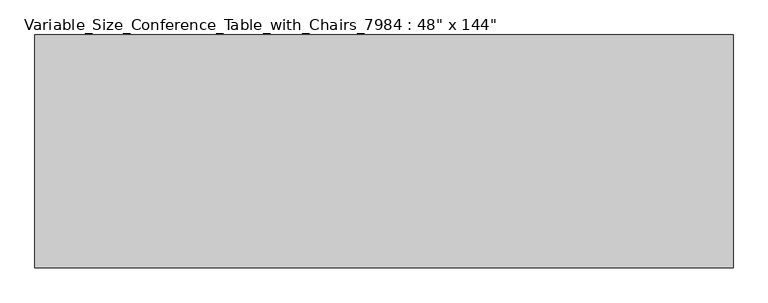
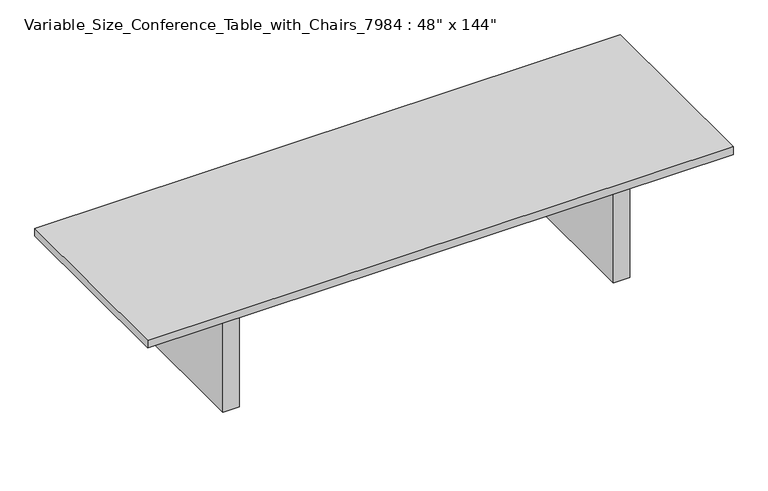
"""IFC4 building model written with IfcOpenShell, lengths in millimetres: furniture geometry."""

from ifc_helpers import new_model, si_unit, frame, origin, origin_with_axes, place, context, project, spatial, polyline, outline, extrude, source, transform, mapped, element, save


def furniture_0c50ee7b(model_context):
    return source(origin(), model_context, "Body", "SweptSolid", [
        extrude(outline(polyline([(1828.8, -609.6), (-1828.8, -609.6), (-1828.8, 609.6), (1828.8, 609.6), (1828.8, -609.6)])), frame((0.0, 0.0, 711.2), z_axis=(0.0, 0.0, 1.0), x_axis=(1.0, 0.0, 0.0)), (0.0, 0.0, 1.0), 50.8),
        extrude(outline(polyline([(1168.4, 457.2), (1168.4, 419.1), (-1168.4, 419.1), (-1168.4, 457.2), (1168.4, 457.2)])), frame((0.0, 0.0, 609.6), z_axis=(0.0, 0.0, 1.0), x_axis=(1.0, 0.0, 0.0)), (0.0, 0.0, 1.0), 101.6),
        extrude(outline(polyline([(1168.4, -457.2), (-1168.4, -457.2), (-1168.4, -419.1), (1168.4, -419.1), (1168.4, -457.2)])), frame((0.0, 0.0, 609.6), z_axis=(0.0, 0.0, 1.0), x_axis=(1.0, 0.0, 0.0)), (0.0, 0.0, 1.0), 101.6),
        extrude(outline(polyline([(-1168.4, -457.2), (-1270.0, -457.2), (-1270.0, 457.2), (-1168.4, 457.2), (-1168.4, -457.2)])), origin_with_axes(), (0.0, 0.0, 1.0), 711.2),
        extrude(outline(polyline([(1270.0, -457.2), (1168.4, -457.2), (1168.4, 457.2), (1270.0, 457.2), (1270.0, -457.2)])), origin_with_axes(), (0.0, 0.0, 1.0), 711.2),
    ])


if __name__ == "__main__":
    model = new_model("IFC4")
    model_context = context("Model", 3, world=origin())
    ifc_project = project(units=[si_unit("LENGTHUNIT", "METRE", prefix="MILLI")], contexts=[model_context])
    site = spatial("IfcSite", under=ifc_project)
    building = spatial("IfcBuilding", under=site)
    placement = place(None, origin())
    furniture_shape = furniture_0c50ee7b(model_context)
    element("IfcFurniture", 1, ObjectType="Variable_Size_Conference_Table_with_Chairs_7984 : 48\" x 144\"", at=placement, inside=building, context=model_context, shape_type="MappedRepresentation", body=[
        mapped(furniture_shape, transform((0.0, 0.0, 0.0), x_axis=(1.0, 0.0, 0.0), y_axis=(0.0, 1.0, 0.0), z_axis=(0.0, 0.0, 1.0))),
    ])
    save(model, "model.ifc")

# Revit data of these elements
# Type "Variable_Size_Conference_Table_with_Chairs_7984 : 48\" x 144\""
#   Model = "353467547"
#   Manufacturer = "Irish Seating"
#   COBie.Type.CreatedBy = "design@eagle.com"
#   COBie.Type.CreatedOn = "2016-09-13T05:47:35"
#   COBie.Type.Name = "Furniture_Variable_Size_Conference_Table_with_Chairs_7984_48\" x 144\""
#   COBie.Type.Category = "23-40 70 14 64 11 : Office Furniture"
#   COBie.Type.Description = "Conference Table Seating 12-14"
#   COBie.Type.Manufacturer = "Irish Seating"
#   COBie.Type.ModelNumber = "353467547"
#   Assembly Code = "E2020200"
#   Description = "Conference Table Seating 12-14"
#   COBie.Type.ReplacementCost = 0
#   Number of Chairs = 0
#   Height = 762 mm
#   Length = 3657.6 mm
#   Width = 1219.2 mm
#   COBie.Type = yes
#   8 Chair = yes
#   14 Chair = no
#   12 Chair = no
#   10 Chair = yes
#   Material = Wood - Cherry
# Element 1 (IfcFurniture, "Variable_Size_Conference_Table_with_Chairs_7984 : 48\" x 144\"")
#   Materials on its faces: "Wood - Cherry"
# Materials
#   "Wood - Cherry": class "Wood", colour RGB 226 177 128, transparency 0
